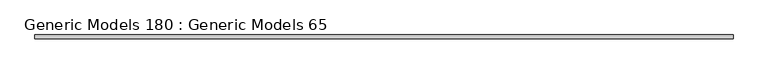
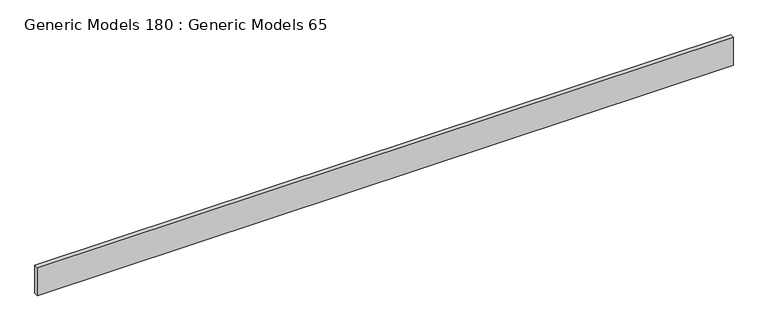
"""IFC4 building model written with IfcOpenShell, lengths in millimetres: proxy geometry, Generic Models 180 : Generic Models 65."""

from ifc_helpers import new_model, si_unit, frame, origin, place, context, project, spatial, polyline, outline, extrude, source, transform, mapped, element, save


def generic_models_180_generic_models_65_71e6eb0b(model_context):
    return source(origin(), model_context, "Body", "SweptSolid", [
        extrude(outline(polyline([(53732.1125, 528.6375), (53732.1125, 547.6875), (57021.4125, 547.6875), (57021.4125, 528.6375), (53732.1125, 528.6375)])), frame((0.0, 0.0, 1612.9), z_axis=(0.0, 0.0, 1.0), x_axis=(1.0, 0.0, 0.0)), (0.0, 0.0, 1.0), 139.7),
    ])


if __name__ == "__main__":
    model = new_model("IFC4")
    model_context = context("Model", 3, world=origin())
    ifc_project = project(units=[si_unit("LENGTHUNIT", "METRE", prefix="MILLI")], contexts=[model_context])
    site = spatial("IfcSite", under=ifc_project)
    building = spatial("IfcBuilding", under=site)
    placement = place(None, origin())
    generic_models_180_generic_models_65_shape = generic_models_180_generic_models_65_71e6eb0b(model_context)
    element("IfcBuildingElementProxy", 1, Name="Generic Models 180 : Generic Models 65", ObjectType="Generic Models 180 : Generic Models 65", at=placement, inside=building, context=model_context, shape_type="MappedRepresentation", body=[
        mapped(generic_models_180_generic_models_65_shape, transform((0.0, 0.0, 0.0), x_axis=(1.0, 0.0, 0.0), y_axis=(0.0, 1.0, 0.0), z_axis=(0.0, 0.0, 1.0))),
    ])
    save(model, "model.ifc")

# Revit data of these elements
# Element 1 (IfcBuildingElementProxy, "Generic Models 180 : Generic Models 65")
#   Materials on its faces: "HORIZONTAL 1X6 CEDAR PLANKS W/ CLEAR WOOD SEALER"
# Materials
#   "HORIZONTAL 1X6 CEDAR PLANKS W/ CLEAR WOOD SEALER": class "Wood", colour RGB 234 198 147, transparency 0, Description = "Pinus Echinata", Cost = 0
